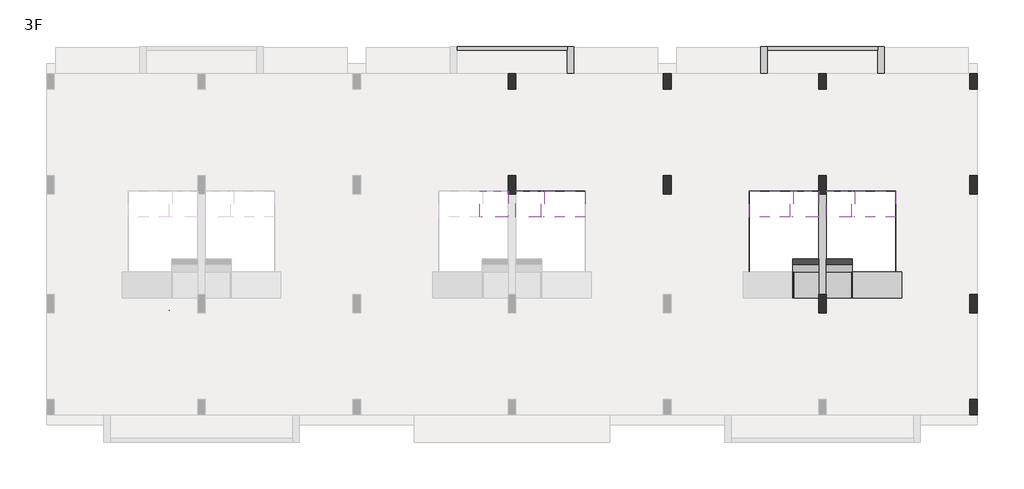
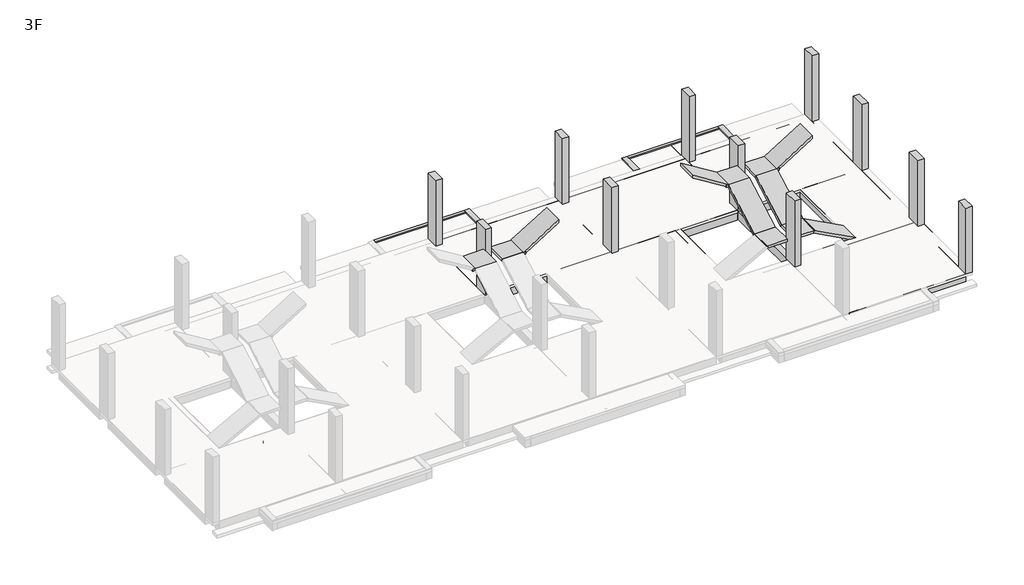
# One storey, part 3 of 3: 36 beams, 11 columns, 1 proxy.
"""IFC4 building model written with IfcOpenShell, lengths in millimetres."""

import ifcopenshell
import ifcopenshell.guid

model = None  # the IFC model being written
_history = None  # IfcOwnerHistory: only IFC2X3 demands one
_inside = {}  # id of a spatial element -> (the spatial element, [elements in it])
_under = {}  # id of a project, library or spatial element -> (it, [spatial elements below it])
_declared = {}  # id of a project -> (the project, [libraries it declares])
_typed = {}  # id of a type object -> (the type object, [elements of that type])
_made_of = {}  # id of a material, layer set ... -> (it, [elements and type objects made of it])


def new_model(schema):
    """Start an empty IFC model of exactly this schema.

    Asked for "IFC4X3", IfcOpenShell would pick the latest addendum, in which some entities
    have other attributes; the version numbers below select the first issue.
    IFC2X3 requires an IfcOwnerHistory on every rooted entity: one is made here for all.
    """
    global model, _history
    if schema == "IFC4X3":
        model = ifcopenshell.file(schema_version=(4, 3, 0, 0))
    else:
        model = ifcopenshell.file(schema=schema)
    _inside.clear()
    _under.clear()
    _declared.clear()
    _typed.clear()
    _made_of.clear()
    _history = None
    if model.schema == "IFC2X3":
        org = make("IfcOrganization", Name="unknown")
        user = make(
            "IfcPersonAndOrganization",
            ThePerson=make("IfcPerson", FamilyName="unknown"),
            TheOrganization=org,
        )
        app = make(
            "IfcApplication",
            ApplicationDeveloper=org,
            Version="unknown",
            ApplicationFullName="unknown",
            ApplicationIdentifier="unknown",
        )
        _history = make(
            "IfcOwnerHistory",
            OwningUser=user,
            OwningApplication=app,
            ChangeAction="ADDED",
            CreationDate=0,
        )
    return model


def make(cls, **values):
    """One entity of the class cls with the attributes given. An attribute that is None is left unset."""
    return model.create_entity(
        cls, **{name: value for name, value in values.items() if value is not None}
    )


def rooted(cls, **values):
    """An entity with a GlobalId (a new one), such as an element, a storey or a relation."""
    return make(cls, GlobalId=ifcopenshell.guid.new(), OwnerHistory=_history, **values)


def si_unit(unit_type, name, prefix=None):
    """IfcSIUnit, for example si_unit("LENGTHUNIT", "METRE", prefix="MILLI")."""
    return make("IfcSIUnit", UnitType=unit_type, Prefix=prefix, Name=name)


def assignment(units):
    """IfcUnitAssignment: the units of a project."""
    return None if units is None else make("IfcUnitAssignment", Units=units)


def point(xyz):
    """IfcCartesianPoint."""
    return None if xyz is None else make("IfcCartesianPoint", Coordinates=xyz)


def direction(xyz):
    """IfcDirection."""
    return None if xyz is None else make("IfcDirection", DirectionRatios=xyz)


def frame(location, z_axis=None, x_axis=None):
    """IfcAxis2Placement3D, a coordinate frame: its origin and axes. An axis left out is left unset."""
    return make(
        "IfcAxis2Placement3D",
        Location=point(location),
        Axis=direction(z_axis),
        RefDirection=direction(x_axis),
    )


def frame_2d(location, x_axis=None):
    """IfcAxis2Placement2D, a coordinate frame in the plane: its origin and x axis."""
    return make(
        "IfcAxis2Placement2D", Location=point(location), RefDirection=direction(x_axis)
    )


def origin():
    """The frame at (0, 0, 0) with its axes left unset."""
    return frame((0.0, 0.0, 0.0))


def origin_with_axes():
    """The frame at (0, 0, 0) with the z axis (0, 0, 1) and the x axis (1, 0, 0) written out."""
    return frame((0.0, 0.0, 0.0), z_axis=(0.0, 0.0, 1.0), x_axis=(1.0, 0.0, 0.0))


def place(relative_to, where):
    """IfcLocalPlacement: puts the frame where relative to a parent placement (None: the world)."""
    return make(
        "IfcLocalPlacement", PlacementRelTo=relative_to, RelativePlacement=where
    )


def context(
    kind, dimensions, precision=None, world=None, true_north=None, identifier=None
):
    """IfcGeometricRepresentationContext, for example the 3D "Model" context."""
    return make(
        "IfcGeometricRepresentationContext",
        ContextIdentifier=identifier,
        ContextType=kind,
        CoordinateSpaceDimension=dimensions,
        Precision=precision,
        WorldCoordinateSystem=world,
        TrueNorth=true_north,
    )


def project(units=None, contexts=None):
    """IfcProject with its units and contexts."""
    return rooted(
        "IfcProject",
        Name="project",
        RepresentationContexts=contexts,
        UnitsInContext=assignment(units),
    )


def spatial(cls, under=None, at=None, **own):
    """A site, building, storey or space (cls), placed at a placement, below another one or the project."""
    s = rooted(cls, ObjectPlacement=at, **own)
    if under is not None:
        _under.setdefault(under.id(), (under, []))[1].append(s)
    return s


def polyline(points):
    """IfcPolyline through the points."""
    return make("IfcPolyline", Points=[point(p) for p in points])


def circle_curve(where, radius):
    """IfcCircle in the frame where."""
    return make("IfcCircle", Position=where, Radius=radius)


def ellipse_curve(where, semi_axis1, semi_axis2):
    """IfcEllipse in the frame where."""
    return make(
        "IfcEllipse", Position=where, SemiAxis1=semi_axis1, SemiAxis2=semi_axis2
    )


def trimmed(basis, trim1, trim2, sense, master):
    """IfcTrimmedCurve: the piece of a basis curve between two trims."""
    return make(
        "IfcTrimmedCurve",
        BasisCurve=basis,
        Trim1=trim1,
        Trim2=trim2,
        SenseAgreement=sense,
        MasterRepresentation=master,
    )


def segment(curve, same_sense, transition):
    """IfcCompositeCurveSegment."""
    return make(
        "IfcCompositeCurveSegment",
        Transition=transition,
        SameSense=same_sense,
        ParentCurve=curve,
    )


def composite_curve(segments, self_intersect=None):
    """IfcCompositeCurve: segments joined end to end."""
    return make("IfcCompositeCurve", Segments=segments, SelfIntersect=self_intersect)


def outline(outer, holes=None, kind="AREA"):
    """IfcArbitraryClosedProfileDef: a profile drawn as a closed curve; with holes, ...WithVoids."""
    if holes is None:
        return make("IfcArbitraryClosedProfileDef", ProfileType=kind, OuterCurve=outer)
    return make(
        "IfcArbitraryProfileDefWithVoids",
        ProfileType=kind,
        OuterCurve=outer,
        InnerCurves=holes,
    )


def extrude(swept, where, along, depth):
    """IfcExtrudedAreaSolid: the profile swept, set in the frame where, extruded along a direction by depth."""
    return make(
        "IfcExtrudedAreaSolid",
        SweptArea=swept,
        Position=where,
        ExtrudedDirection=direction(along),
        Depth=depth,
    )


def faces_of(points, faces, orient=None, outer=None):
    """IfcFace entities. A face is a list of loops; a loop is a list of indices into points, from 0.

    orient and outer hold one flag for each loop. By default every Orientation is true, the
    first loop of a face is its IfcFaceOuterBound and the others are IfcFaceBound.
    """
    made = []
    for i, loops in enumerate(faces):
        bounds = []
        for j, loop in enumerate(loops):
            is_outer = j == 0 if outer is None else outer[i][j]
            bounds.append(
                make(
                    "IfcFaceOuterBound" if is_outer else "IfcFaceBound",
                    Bound=make("IfcPolyLoop", Polygon=[points[k] for k in loop]),
                    Orientation=True if orient is None else orient[i][j],
                )
            )
        made.append(make("IfcFace", Bounds=bounds))
    return made


def faceted_brep(points, faces, orient=None, outer=None, voids=None):
    """IfcFacetedBrep: a solid bounded by flat faces; with voids (closed shells), ...WithVoids."""
    shared = [point(p) for p in points]
    hull = make("IfcClosedShell", CfsFaces=faces_of(shared, faces, orient, outer))
    if voids is None:
        return make("IfcFacetedBrep", Outer=hull)
    return make(
        "IfcFacetedBrepWithVoids",
        Outer=hull,
        Voids=[
            make(cls, CfsFaces=faces_of(shared, fs, o, b)) for cls, fs, o, b in voids
        ],
    )


def shape(context_of_items, identifier, shape_type, items):
    """IfcShapeRepresentation: the items that make up one representation, for example the "Body"."""
    return make(
        "IfcShapeRepresentation",
        ContextOfItems=context_of_items,
        RepresentationIdentifier=identifier,
        RepresentationType=shape_type,
        Items=items,
    )


def source(mapping_origin, context_of_items, identifier, shape_type, items):
    """IfcRepresentationMap: a shape defined once, which mapped items show again and again."""
    return make(
        "IfcRepresentationMap",
        MappingOrigin=mapping_origin,
        MappedRepresentation=shape(context_of_items, identifier, shape_type, items),
    )


def transform(
    local_origin,
    x_axis=None,
    y_axis=None,
    z_axis=None,
    scale=None,
    scale2=None,
    scale3=None,
    uniform=True,
):
    """IfcCartesianTransformationOperator3D, or its non-uniform kind. x_axis, y_axis, z_axis: its Axis1, 2, 3."""
    if uniform:
        return make(
            "IfcCartesianTransformationOperator3D",
            Axis1=direction(x_axis),
            Axis2=direction(y_axis),
            LocalOrigin=point(local_origin),
            Scale=scale,
            Axis3=direction(z_axis),
        )
    return make(
        "IfcCartesianTransformationOperator3DnonUniform",
        Axis1=direction(x_axis),
        Axis2=direction(y_axis),
        LocalOrigin=point(local_origin),
        Scale=scale,
        Axis3=direction(z_axis),
        Scale2=scale2,
        Scale3=scale3,
    )


def mapped(mapping_source, mapping_target):
    """IfcMappedItem: shows the shape of a source again, moved by a transform."""
    return make(
        "IfcMappedItem", MappingSource=mapping_source, MappingTarget=mapping_target
    )


def made_of(thing, what):
    """Note that an element or type object is made of a material, layer set ...; save() writes the relation."""
    if what is not None:
        _made_of.setdefault(what.id(), (what, []))[1].append(thing)
    return thing


def element(
    cls,
    number,
    at=None,
    inside=None,
    cuts=None,
    type_object=None,
    material=None,
    context=None,
    identifier="Body",
    shape_type=None,
    held_by="IfcProductDefinitionShape",
    body=None,
    shapes=None,
    **own,
):
    """One element of the class cls, such as IfcWall. Its Tag is "e" and its number.

    at: its placement. inside: the storey or other place that contains it. cuts: it is an
    opening in that element (IfcRelVoidsElement). A single representation is given by context,
    identifier, shape_type and body (its items); several are given by shapes. held_by: the class
    of the entity that holds the representations. save() writes the other relations.
    """
    e = rooted(cls, Tag="e%d" % number, ObjectPlacement=at, **own)
    if body is not None:
        shapes = [shape(context, identifier, shape_type, body)]
    if shapes is not None:
        e.Representation = make(held_by, Representations=shapes)
    if inside is not None:
        _inside.setdefault(inside.id(), (inside, []))[1].append(e)
    if cuts is not None:
        rooted(
            "IfcRelVoidsElement", RelatingBuildingElement=cuts, RelatedOpeningElement=e
        )
    if type_object is not None:
        _typed.setdefault(type_object.id(), (type_object, []))[1].append(e)
    return made_of(e, material)


def aggregate(whole, parts):
    """IfcRelAggregates: a whole, such as a stair, and the parts it consists of."""
    return rooted("IfcRelAggregates", RelatingObject=whole, RelatedObjects=parts)


def save(model, path):
    """Write the relations noted so far, then the file.

    IfcRelAggregates (storeys below a building ...), IfcRelContainedInSpatialStructure (elements
    in a storey), IfcRelDefinesByType, IfcRelAssociatesMaterial and IfcRelDeclares: one each for
    every whole, place, type object, material and project.
    """
    for whole, parts in _under.values():
        aggregate(whole, parts)
    for where, things in _inside.values():
        rooted(
            "IfcRelContainedInSpatialStructure",
            RelatedElements=things,
            RelatingStructure=where,
        )
    for kind, things in _typed.values():
        rooted("IfcRelDefinesByType", RelatedObjects=things, RelatingType=kind)
    for what, things in _made_of.values():
        rooted("IfcRelAssociatesMaterial", RelatedObjects=things, RelatingMaterial=what)
    for by, libraries in _declared.values():
        rooted("IfcRelDeclares", RelatingContext=by, RelatedDefinitions=libraries)
    model.write(path)


def plane_surface(at):
    """IfcPlane: the flat surface through the origin of the frame at, square to its z axis."""
    return make("IfcPlane", Position=at)


def cylinder_surface(at, radius):
    """IfcCylindricalSurface: all points at the distance radius from the z axis of the frame at."""
    return make("IfcCylindricalSurface", Position=at, Radius=radius)


def revolved_surface(curve, axis_point, axis_direction):
    """IfcSurfaceOfRevolution: the curve turned about the line through axis_point along axis_direction."""
    return make(
        "IfcSurfaceOfRevolution",
        SweptCurve=make("IfcArbitraryOpenProfileDef", ProfileType="CURVE", Curve=curve),
        AxisPosition=make("IfcAxis1Placement", Location=point(axis_point), Axis=direction(axis_direction)),
    )


def advanced_brep(points, edges, surfaces, faces):
    """IfcAdvancedBrep: a solid bounded by faces that lie on surfaces and meet in shared edges.

    An edge is (start, end): straight between two places in points (the first is 0);
    or (start, end, curve); or (start, end, curve, False) where it runs against its curve.
    A face is (place in surfaces, loops), or (place, loops, False) where it looks against
    its surface's normal. A loop lists edges by number (the first is 1), with a minus sign
    where the edge is run from its end to its start. The first loop is the outer one.
    """
    corners = [point(p) for p in points]
    vertices = [make("IfcVertexPoint", VertexGeometry=c) for c in corners]
    made = []
    for start, end, *more in edges:
        made.append(
            make(
                "IfcEdgeCurve",
                EdgeStart=vertices[start],
                EdgeEnd=vertices[end],
                EdgeGeometry=more[0] if more else make("IfcPolyline", Points=[corners[start], corners[end]]),
                SameSense=more[1] if len(more) > 1 else True,
            )
        )
    hull = []
    for where, loops, *sense in faces:
        bounds = []
        for j, loop in enumerate(loops):
            ring = [make("IfcOrientedEdge", EdgeElement=made[abs(k) - 1], Orientation=k > 0) for k in loop]
            bounds.append(
                make(
                    "IfcFaceOuterBound" if j == 0 else "IfcFaceBound",
                    Bound=make("IfcEdgeLoop", EdgeList=ring),
                    Orientation=True,
                )
            )
        hull.append(make("IfcAdvancedFace", Bounds=bounds, FaceSurface=surfaces[where], SameSense=sense[0] if sense else True))
    return make("IfcAdvancedBrep", Outer=make("IfcClosedShell", CfsFaces=hull))


def m_support_metal_circular_m_support_metal_circular_a779fbb7(model_context):
    return source(origin(), model_context, "Body", "SolidModel", [
        advanced_brep(
        [(-6.0, 0.0, 0.0), (6.0, 0.0, 0.0), (-6.0, 0.0, -63.0), (6.0, 0.0, -63.0), (6.0, 12.0, -75.0), (-6.0, 12.0, -75.0), (-6.0, 63.0, -75.0), (6.0, 63.0, -75.0)],
        [
            (0, 1, circle_curve(origin_with_axes(), 6.0)),
            (1, 0, circle_curve(origin_with_axes(), 6.0)),
            (0, 2),
            (2, 3, circle_curve(frame((0.0, 0.0, -63.0), z_axis=(0.0, 0.0, 1.0), x_axis=(1.0, 0.0, 0.0)), 6.0)),
            (3, 1),
            (3, 2, circle_curve(frame((0.0, 0.0, -63.0), z_axis=(0.0, 0.0, 1.0), x_axis=(1.0, 0.0, 0.0)), 6.0)),
            (4, 3, circle_curve(frame((6.0, 12.0, -63.0), z_axis=(-1.0, 0.0, 0.0), x_axis=(0.0, -1.0, 0.0)), 12.0)),
            (2, 5, circle_curve(frame((-6.0, 12.0, -63.0), z_axis=(1.0, 0.0, 0.0), x_axis=(0.0, -1.0, 0.0)), 12.0)),
            (5, 4, circle_curve(frame((0.0, 12.0, -75.0), z_axis=(0.0, -1.0, 0.0), x_axis=(1.0, 0.0, 0.0)), 6.0)),
            (4, 5, circle_curve(frame((0.0, 12.0, -75.0), z_axis=(0.0, -1.0, 0.0), x_axis=(1.0, 0.0, 0.0)), 6.0)),
            (6, 7, circle_curve(frame((0.0, 63.0, -75.0), z_axis=(0.0, 1.0, 0.0), x_axis=(1.0, 0.0, 0.0)), 6.0)),
            (7, 6, circle_curve(frame((0.0, 63.0, -75.0), z_axis=(0.0, 1.0, 0.0), x_axis=(1.0, 0.0, 0.0)), 6.0)),
            (5, 6),
            (7, 4),
        ],
        [
            plane_surface(origin_with_axes()),
            cylinder_surface(origin_with_axes(), 6.0),
            revolved_surface(trimmed(ellipse_curve(frame((0.0, 0.0, -63.0), z_axis=(0.0, 0.0, 1.0), x_axis=(1.0, 0.0, 0.0)), 6.0, 6.0), [point((-6.0, 0.0, -63.0))], [point((6.0, 0.0, -63.0))], True, "CARTESIAN"), (0.0, 12.0, -63.0), (1.0, 0.0, 0.0)),
            revolved_surface(trimmed(ellipse_curve(frame((0.0, 0.0, -63.0), z_axis=(0.0, 0.0, 1.0), x_axis=(1.0, 0.0, 0.0)), 6.0, 6.0), [point((6.0, 0.0, -63.0))], [point((-6.0, 0.0, -63.0))], True, "CARTESIAN"), (0.0, 12.0, -63.0), (1.0, 0.0, 0.0)),
            plane_surface(frame((0.0, 63.0, -75.0), z_axis=(0.0, 1.0, 0.0), x_axis=(1.0, 0.0, 0.0))),
            cylinder_surface(frame((0.0, 12.0, -75.0), z_axis=(0.0, -1.0, 0.0), x_axis=(1.0, 0.0, 0.0)), 6.0),
        ],
        [
            (0, [[1, 2]]),
            (1, [[-1, 3, 4, 5]]),
            (1, [[-2, -5, 6, -3]]),
            (2, [[7, -4, 8, 9]]),
            (3, [[-8, -6, -7, 10]]),
            (4, [[11, 12]]),
            (5, [[-9, 13, -12, 14]]),
            (5, [[-10, -14, -11, -13]]),
        ],
    ),
        extrude(outline(composite_curve([segment(trimmed(circle_curve(frame_2d((-75.0, 0.0)), 25.0), [point((-75.0, -25.0))], [point((-75.0, 25.0))], False, "CARTESIAN"), True, "CONTINUOUS"), segment(trimmed(circle_curve(frame_2d((-75.0, 0.0)), 25.0), [point((-75.0, 25.0))], [point((-75.0, -25.0))], False, "CARTESIAN"), True, "CONTINUOUS")], self_intersect=False)), frame((0.0, 63.0, 0.0), z_axis=(0.0, 1.0, 0.0), x_axis=(0.0, 0.0, 1.0)), (0.0, 0.0, 1.0), 12.0),
    ])


model = new_model("IFC4")

# Units and contexts
model_context = context("Model", 3, world=origin())
ifc_project = project(units=[si_unit("LENGTHUNIT", "METRE", prefix="MILLI")], contexts=[model_context])

# Site, building, storey
site = spatial("IfcSite", under=ifc_project)
building = spatial("IfcBuilding", under=site)
storey = spatial("IfcBuildingStorey", under=building, Name="3F", Elevation=7330.0)

# Beams
placement = place(None, origin())
element("IfcBeam", 1, ObjectType="M_Concrete-Rectangular Beam : 1000x120", at=placement, inside=storey, context=model_context, shape_type="Brep", body=[
    faceted_brep([(16600.0000058, 7550.0000002, 9580.0), (16600.0000058, 8550.0000002, 9580.0), (16600.0000058, 8550.0000002, 9460.0), (16600.0000058, 7550.0000002, 9460.0), (17700.0000058, 8550.0000002, 9460.0), (17700.0000058, 8550.0000002, 9580.0), (17700.0000058, 7550.0000002, 9580.0), (17700.0000058, 7609.0063595, 9475.5095719), (17700.0000058, 7581.5414925, 9460.0), (16700.0000058, 7550.0000002, 9580.0), (16700.0000058, 7581.5414925, 9460.0), (16700.0000058, 7550.0000002, 9460.0), (16700.0000058, 7609.0063595, 9475.5095719)], [[[0, 1, 2, 3]], [[4, 5, 6, 7, 8]], [[1, 0, 9, 6, 5]], [[2, 1, 5, 4]], [[3, 2, 4, 8, 10, 11]], [[0, 3, 11, 9]], [[12, 7, 6, 9]], [[7, 12, 10, 8]], [[12, 9, 11, 10]]]),
])
element("IfcBeam", 2, ObjectType="M_Concrete-Rectangular Beam : 1000x120", at=placement, inside=storey, context=model_context, shape_type="Brep", body=[
    faceted_brep([(19100.0000058, 8550.0000002, 9580.0), (19100.0000058, 7550.0000002, 9580.0), (19100.0000058, 7550.0000002, 9460.0), (19100.0000058, 8550.0000002, 9460.0), (18000.0000058, 8550.0000002, 9580.0), (18000.0000058, 8550.0000002, 9460.0), (18000.0000058, 7581.5414925, 9460.0), (18000.0000058, 7609.0063595, 9475.5095719), (18000.0000058, 7550.0000002, 9580.0), (19000.0000058, 7550.0000002, 9580.0), (19000.0000058, 7550.0000002, 9460.0), (19000.0000058, 7581.5414925, 9460.0), (19000.0000058, 7609.0063595, 9475.5095719)], [[[0, 1, 2, 3]], [[4, 5, 6, 7, 8]], [[1, 0, 4, 8, 9]], [[0, 3, 5, 4]], [[3, 2, 10, 11, 6, 5]], [[2, 1, 9, 10]], [[12, 9, 8, 7]], [[12, 7, 6, 11]], [[9, 12, 11, 10]]]),
])
element("IfcBeam", 3, ObjectType="M_Concrete-Rectangular Beam : 1000x120", at=placement, inside=storey, context=model_context, shape_type="Brep", body=[
    faceted_brep([(18984.2496976, 7549.9999993, 9580.0), (20680.0000464, 7549.9999993, 10630.0), (20680.0000058, 8549.9999993, 10629.9999748), (18984.2496976, 8549.9999993, 9580.0), (20680.0000058, 8549.9999993, 10488.8582241), (19100.0000058, 8549.9999993, 9510.5302519), (19100.0000058, 8549.9999993, 9580.0), (19100.0000058, 7549.9999993, 9510.5302519), (20680.0000058, 7549.9999993, 10488.8582241), (19000.0000058, 7549.9999993, 9580.0), (19100.0000058, 7549.9999993, 9580.0)], [[[0, 1, 2, 3]], [[3, 2, 4, 5, 6]], [[7, 5, 4, 8]], [[1, 0, 9, 10, 7, 8]], [[10, 6, 5, 7]], [[6, 10, 9, 0, 3]], [[2, 1, 8, 4]]]),
])
element("IfcBeam", 4, ObjectType="M_Concrete-Rectangular Beam : 1000x120", at=placement, inside=storey, context=model_context, shape_type="Brep", body=[
    faceted_brep([(28700.0000039, 7550.0000002, 9580.0), (29700.0000039, 7550.0000002, 9580.0), (29700.0000039, 7609.0063595, 9475.5095719), (28700.0000039, 7609.0063595, 9475.5095719), (28700.0000039, 5424.9999998, 8380.0), (28700.0000039, 5484.0063591, 8275.5095719), (29700.0000039, 5484.0063591, 8275.5095719), (29700.0000039, 5424.9999998, 8380.0), (29700.0000039, 5524.9999998, 8298.6589219), (29700.0000039, 7581.5414925, 9460.0), (28700.0000039, 5524.9999998, 8298.6589219), (28700.0000039, 7581.5414925, 9460.0)], [[[0, 1, 2, 3]], [[4, 5, 6, 7]], [[1, 0, 4, 7]], [[2, 1, 7, 6, 8, 9]], [[3, 2, 9, 8, 6, 5, 10, 11]], [[0, 3, 11, 10, 5, 4]]]),
])
element("IfcBeam", 5, ObjectType="M_Concrete-Rectangular Beam : 1000x120", at=placement, inside=storey, context=model_context, shape_type="Brep", body=[
    faceted_brep([(28600.0000039, 7550.0000002, 9580.0), (28600.0000039, 8550.0000002, 9580.0), (28600.0000039, 8550.0000002, 9460.0), (28600.0000039, 7550.0000002, 9460.0), (29700.0000039, 8550.0000002, 9460.0), (29700.0000039, 8550.0000002, 9580.0), (29700.0000039, 7550.0000002, 9580.0), (29700.0000039, 7609.0063595, 9475.5095719), (29700.0000039, 7581.5414925, 9460.0), (28700.0000039, 7550.0000002, 9580.0), (28700.0000039, 7581.5414925, 9460.0), (28700.0000039, 7550.0000002, 9460.0), (28700.0000039, 7609.0063595, 9475.5095719)], [[[0, 1, 2, 3]], [[4, 5, 6, 7, 8]], [[1, 0, 9, 6, 5]], [[2, 1, 5, 4]], [[3, 2, 4, 8, 10, 11]], [[0, 3, 11, 9]], [[12, 7, 6, 9]], [[7, 12, 10, 8]], [[12, 9, 11, 10]]]),
])
element("IfcBeam", 6, ObjectType="M_Concrete-Rectangular Beam : 1000x120", at=placement, inside=storey, context=model_context, shape_type="Brep", body=[
    faceted_brep([(27019.9999632, 7549.9999993, 10630.0), (28715.750312, 7549.9999993, 9580.0), (28715.750312, 8549.9999993, 9580.0), (27019.9999632, 8549.9999993, 10630.0), (28600.0000039, 8549.9999993, 9580.0), (28600.0000039, 8549.9999993, 9510.5302519), (27020.000004, 8549.9999993, 10488.8582239), (28600.0000039, 7549.9999993, 9510.5302519), (27020.000004, 7549.9999993, 10488.8582239), (28600.0000039, 7549.9999993, 9580.0), (28700.0000039, 7549.9999993, 9580.0)], [[[0, 1, 2, 3]], [[3, 2, 4, 5, 6]], [[5, 7, 8, 6]], [[1, 0, 8, 7, 9, 10]], [[4, 9, 7, 5]], [[9, 4, 2, 1, 10]], [[0, 3, 6, 8]]]),
])
element("IfcBeam", 7, ObjectType="M_Concrete-Rectangular Beam : 1000x120", at=placement, inside=storey, context=model_context, shape_type="Brep", body=[
    faceted_brep([(29700.0000039, 5524.9999998, 8260.0), (28700.0000039, 5524.9999998, 8260.0), (28700.0000039, 5524.9999998, 8298.6589219), (29700.0000039, 5524.9999998, 8298.6589219), (29700.0000039, 4424.9999998, 8260.0), (29700.0000039, 4424.9999998, 8380.0), (28730.4772098, 4424.9999998, 8380.0), (28787.1330609, 4424.9999998, 8274.2166623), (28760.5888301, 4424.9999998, 8260.0), (29700.0000039, 5424.9999998, 8380.0), (28700.0000039, 5424.9999998, 8380.0), (28700.0000039, 4424.9999998, 8380.0), (29700.0000039, 5484.0063591, 8275.5095719), (28760.5888301, 5424.9999998, 8260.0), (28700.0000039, 5424.9999998, 8260.0), (28700.0000039, 4424.9999998, 8363.6768996), (28700.0000039, 5484.0063591, 8275.5095719), (28700.0000039, 5424.9999998, 8363.6768996), (28730.4772098, 5424.9999998, 8380.0), (28787.1330609, 5424.9999998, 8274.2166623)], [[[0, 1, 2, 3]], [[4, 5, 6, 7, 8]], [[6, 5, 9, 10, 11]], [[5, 4, 0, 3, 12, 9]], [[1, 0, 4, 8, 13, 14]], [[15, 11, 10, 16, 2, 1, 14, 17]], [[6, 18, 19, 7]], [[18, 6, 15, 17]], [[7, 19, 13, 8]], [[19, 18, 17, 14, 13]], [[11, 15, 6]], [[12, 16, 10, 9]], [[16, 12, 3, 2]]]),
])
element("IfcBeam", 8, ObjectType="M_Concrete-Rectangular Beam : 1000x120", at=placement, inside=storey, context=model_context, shape_type="Brep", body=[
    faceted_brep([(30969.5227979, 4424.9999998, 8380.0), (30969.5227979, 5424.9999998, 8380.0), (30912.8669468, 5424.9999998, 8274.2166623), (30912.8669468, 4424.9999998, 8274.2166623), (31000.0000039, 4424.9999998, 8363.6768996), (32930.0000046, 4424.9999998, 7330.0), (32930.0000046, 5424.9999998, 7330.0), (31000.0000039, 5424.9999998, 8363.6768996), (30939.4111776, 4424.9999998, 8260.0), (32675.8338464, 4424.9999998, 7330.0), (30939.4111776, 5424.9999998, 8260.0), (32680.0000108, 5424.9999998, 7327.7686695), (32680.0000108, 4449.9999998, 7327.7686695), (32675.8338464, 4449.9999998, 7330.0), (32680.0000108, 5424.9999998, 7330.0), (32680.0000108, 4449.9999998, 7330.0)], [[[0, 1, 2, 3]], [[1, 0, 4, 5, 6, 7]], [[0, 3, 8, 9, 5, 4]], [[3, 2, 10, 11, 12, 13, 9, 8]], [[2, 1, 7, 6, 14, 11, 10]], [[9, 13, 15, 14, 6, 5]], [[11, 14, 15, 12]], [[15, 13, 12]]]),
])
element("IfcBeam", 9, ObjectType="M_Concrete-Rectangular Beam : 1000x120", at=placement, inside=storey, context=model_context, shape_type="Brep", body=[
    faceted_brep([(31000.0000039, 7550.0000002, 9580.0), (31000.0000039, 7609.0063595, 9475.5095719), (30000.0000039, 7609.0063595, 9475.5095719), (30000.0000039, 7550.0000002, 9580.0), (31000.0000039, 5424.9999998, 8380.0), (30000.0000039, 5424.9999998, 8380.0), (30000.0000039, 5484.0063591, 8275.5095719), (31000.0000039, 5484.0063591, 8275.5095719), (30000.0000039, 7581.5414925, 9460.0), (30000.0000039, 5524.9999998, 8298.6589219), (31000.0000039, 7581.5414925, 9460.0), (31000.0000039, 5524.9999998, 8298.6589219)], [[[0, 1, 2, 3]], [[4, 5, 6, 7]], [[3, 5, 4, 0]], [[2, 8, 9, 6, 5, 3]], [[1, 10, 11, 7, 6, 9, 8, 2]], [[0, 4, 7, 11, 10, 1]]]),
])
element("IfcBeam", 10, ObjectType="M_Concrete-Rectangular Beam : 1000x120", at=placement, inside=storey, context=model_context, shape_type="Brep", body=[
    faceted_brep([(31100.0000039, 8550.0000002, 9580.0), (31100.0000039, 7550.0000002, 9580.0), (31100.0000039, 7550.0000002, 9460.0), (31100.0000039, 8550.0000002, 9460.0), (30000.0000039, 8550.0000002, 9580.0), (30000.0000039, 8550.0000002, 9460.0), (30000.0000039, 7581.5414925, 9460.0), (30000.0000039, 7609.0063595, 9475.5095719), (30000.0000039, 7550.0000002, 9580.0), (31000.0000039, 7550.0000002, 9580.0), (31000.0000039, 7550.0000002, 9460.0), (31000.0000039, 7581.5414925, 9460.0), (31000.0000039, 7609.0063595, 9475.5095719)], [[[0, 1, 2, 3]], [[4, 5, 6, 7, 8]], [[1, 0, 4, 8, 9]], [[0, 3, 5, 4]], [[3, 2, 10, 11, 6, 5]], [[2, 1, 9, 10]], [[12, 9, 8, 7]], [[12, 7, 6, 11]], [[9, 12, 11, 10]]]),
])
element("IfcBeam", 11, ObjectType="M_Concrete-Rectangular Beam : 1000x120", at=placement, inside=storey, context=model_context, shape_type="Brep", body=[
    faceted_brep([(30984.2496957, 7549.9999993, 9580.0), (32680.0000445, 7549.9999993, 10630.0), (32680.0000108, 8549.9999993, 10629.9999791), (30984.2496957, 8549.9999993, 9580.0), (32680.0000108, 8549.9999993, 10488.8582284), (31100.0000039, 8549.9999993, 9510.5302519), (31100.0000039, 8549.9999993, 9580.0), (31100.0000039, 7549.9999993, 9510.5302519), (32680.0000108, 7549.9999993, 10488.8582284), (31000.0000039, 7549.9999993, 9580.0), (31100.0000039, 7549.9999993, 9580.0)], [[[0, 1, 2, 3]], [[3, 2, 4, 5, 6]], [[7, 5, 4, 8]], [[1, 0, 9, 10, 7, 8]], [[10, 6, 5, 7]], [[6, 10, 9, 0, 3]], [[2, 1, 8, 4]]]),
])
element("IfcBeam", 12, ObjectType="M_Concrete-Rectangular Beam : 1000x120", at=placement, inside=storey, context=model_context, shape_type="Brep", body=[
    faceted_brep([(31000.0000039, 5524.9999998, 8260.0), (30000.0000039, 5524.9999998, 8260.0), (30000.0000039, 5524.9999998, 8298.6589219), (31000.0000039, 5524.9999998, 8298.6589219), (30000.0000039, 4424.9999998, 8380.0), (30000.0000039, 4424.9999998, 8260.0), (30939.4111776, 4424.9999998, 8260.0), (30912.8669468, 4424.9999998, 8274.2166623), (30969.5227979, 4424.9999998, 8380.0), (31000.0000039, 4424.9999998, 8380.0), (31000.0000039, 5424.9999998, 8380.0), (30000.0000039, 5424.9999998, 8380.0), (30000.0000039, 5484.0063591, 8275.5095719), (31000.0000039, 5424.9999998, 8260.0), (30939.4111776, 5424.9999998, 8260.0), (31000.0000039, 4424.9999998, 8363.6768996), (31000.0000039, 5424.9999998, 8363.6768996), (31000.0000039, 5484.0063591, 8275.5095719), (30969.5227979, 5424.9999998, 8380.0), (30912.8669468, 5424.9999998, 8274.2166623)], [[[0, 1, 2, 3]], [[4, 5, 6, 7, 8]], [[8, 9, 10, 11, 4]], [[5, 4, 11, 12, 2, 1]], [[1, 0, 13, 14, 6, 5]], [[9, 15, 16, 13, 0, 3, 17, 10]], [[18, 8, 7, 19]], [[8, 18, 16, 15]], [[19, 7, 6, 14]], [[18, 19, 14, 13, 16]], [[15, 9, 8]], [[17, 12, 11, 10]], [[12, 17, 3, 2]]]),
])
element("IfcBeam", 13, ObjectType="M_Concrete-Rectangular Beam : 150x500", at=placement, inside=storey, context=model_context, shape_type="SweptSolid", body=[
    extrude(outline(polyline([(19989.9825383, 14150.0000066), (19989.9825383, 14000.0000066), (15710.0998466, 14000.0000066), (15710.0998466, 14150.0000066), (19989.9825383, 14150.0000066)])), frame((0.0, 0.0, 6830.0), z_axis=(0.0, 0.0, 1.0), x_axis=(1.0, 0.0, 0.0)), (0.0, 0.0, 1.0), 500.0),
])
element("IfcBeam", 14, ObjectType="M_Concrete-Rectangular Beam : 150x500", at=placement, inside=storey, context=model_context, shape_type="SweptSolid", body=[
    extrude(outline(polyline([(31989.900241, 14150.0000066), (31989.900241, 14000.0000066), (27710.0128711, 14000.0000066), (27710.0128711, 14150.0000066), (31989.900241, 14150.0000066)])), frame((0.0, 0.0, 6830.0), z_axis=(0.0, 0.0, 1.0), x_axis=(1.0, 0.0, 0.0)), (0.0, 0.0, 1.0), 500.0),
])
element("IfcBeam", 15, ObjectType="M_Concrete-Rectangular Beam : 250x400", at=placement, inside=storey, context=model_context, shape_type="Brep", body=[
    faceted_brep([(32930.0000108, 8549.9999993, 7330.0), (32680.0000108, 8549.9999993, 7330.0), (32680.0000108, 5424.9999998, 7330.0), (32680.0000108, 4449.9999998, 7330.0), (32930.0000108, 4449.9999998, 7330.0), (32930.0000108, 8549.9999993, 6930.0), (32930.0000108, 4449.9999998, 6930.0), (32680.0000108, 8549.9999993, 6930.0), (32680.0000108, 4449.9999998, 6930.0), (32680.0000108, 8549.9999993, 7188.8582284), (32680.0000108, 4449.9999998, 7327.7686695)], [[[0, 1, 2, 3, 4]], [[5, 0, 4, 6]], [[7, 5, 6, 8]], [[1, 9, 7, 8, 10, 3, 2]], [[1, 0, 5, 7, 9]], [[4, 3, 10, 8, 6]]]),
])
element("IfcBeam", 16, ObjectType="M_Concrete-Rectangular Beam : 250x400", at=placement, inside=storey, context=model_context, shape_type="Brep", body=[
    faceted_brep([(27020.000004, 8549.9999993, 7330.0), (26770.000004, 8549.9999993, 7330.0), (26770.000004, 4449.9999998, 7330.0), (27020.000004, 4449.9999998, 7330.0), (27020.000004, 5424.9999998, 7330.0), (27020.000004, 8549.9999993, 6930.0), (27020.000004, 8549.9999993, 7188.8582239), (27020.000004, 4449.9999998, 7327.7686733), (27020.000004, 4449.9999998, 6930.0), (26770.000004, 8549.9999993, 6930.0), (26770.000004, 4449.9999998, 6930.0)], [[[0, 1, 2, 3, 4]], [[5, 6, 0, 4, 3, 7, 8]], [[9, 5, 8, 10]], [[1, 9, 10, 2]], [[1, 0, 6, 5, 9]], [[3, 2, 10, 8, 7]]]),
])
element("IfcBeam", 17, ObjectType="M_Concrete-Rectangular Beam : 250x500", at=placement, inside=storey, context=model_context, shape_type="Brep", body=[
    faceted_brep([(20239.9825383, 14150.0000066, 7330.0), (19989.9825383, 14150.0000066, 7330.0), (19989.9825383, 14000.0000066, 7330.0), (19989.9825383, 13100.0000001, 7330.0), (20239.9825383, 13100.0000001, 7330.0), (19989.9825383, 14150.0000066, 6830.0), (19989.9825383, 14000.0000066, 6830.0), (19989.9825383, 13100.0000001, 6830.0), (20239.9825383, 14150.0000066, 6830.0), (20239.9825383, 13100.0000001, 6830.0)], [[[0, 1, 2, 3, 4]], [[1, 5, 6, 7, 3, 2]], [[5, 8, 9, 7, 6]], [[8, 0, 4, 9]], [[1, 0, 8, 5]], [[4, 3, 7, 9]]]),
])
element("IfcBeam", 18, ObjectType="M_Concrete-Rectangular Beam : 250x500", at=placement, inside=storey, context=model_context, shape_type="Brep", body=[
    faceted_brep([(32239.900241, 14150.0000066, 7330.0), (31989.900241, 14150.0000066, 7330.0), (31989.900241, 14000.0000066, 7330.0), (31989.900241, 13100.0000001, 7330.0), (32239.900241, 13100.0000001, 7330.0), (31989.900241, 14150.0000066, 6830.0), (31989.900241, 14000.0000066, 6830.0), (31989.900241, 13100.0000001, 6830.0), (32239.900241, 14150.0000066, 6830.0), (32239.900241, 13100.0000001, 6830.0)], [[[0, 1, 2, 3, 4]], [[1, 5, 6, 7, 3, 2]], [[5, 8, 9, 7, 6]], [[8, 0, 4, 9]], [[4, 3, 7, 9]], [[1, 0, 8, 5]]]),
])
element("IfcBeam", 19, ObjectType="M_Concrete-Rectangular Beam : 250x500", at=placement, inside=storey, context=model_context, shape_type="Brep", body=[
    faceted_brep([(27710.0128711, 14150.0000066, 7330.0), (27460.0128711, 14150.0000066, 7330.0), (27460.0128711, 13100.0000001, 7330.0), (27710.0128711, 13100.0000001, 7330.0), (27710.0128711, 14000.0000066, 7330.0), (27710.0128711, 14150.0000066, 6830.0), (27710.0128711, 13100.0000001, 6830.0), (27710.0128711, 14000.0000066, 6830.0), (27460.0128711, 14150.0000066, 6830.0), (27460.0128711, 13100.0000001, 6830.0)], [[[0, 1, 2, 3, 4]], [[5, 0, 4, 3, 6, 7]], [[8, 5, 7, 6, 9]], [[1, 8, 9, 2]], [[3, 2, 9, 6]], [[1, 0, 5, 8]]]),
])
element("IfcBeam", 20, ObjectType="M_Concrete-Rectangular Beam : 300x400", at=placement, inside=storey, context=model_context, shape_type="SweptSolid", body=[
    extrude(outline(polyline([(18000.0000046, 9150.0), (17700.0000046, 9150.0), (17700.0000046, 12500.0000003), (18000.0000046, 12500.0000003), (18000.0000046, 9150.0)])), frame((0.0, 0.0, 6930.0), z_axis=(0.0, 0.0, 1.0), x_axis=(1.0, 0.0, 0.0)), (0.0, 0.0, 1.0), 400.0),
])
element("IfcBeam", 21, ObjectType="M_Concrete-Rectangular Beam : 300x400", at=placement, inside=storey, context=model_context, shape_type="SweptSolid", body=[
    extrude(outline(polyline([(30000.0000031, 9149.9985388), (29700.0000031, 9149.9985388), (29700.0000031, 12500.0000003), (30000.0000031, 12500.0000003), (30000.0000031, 9149.9985388)])), frame((0.0, 0.0, 6930.0), z_axis=(0.0, 0.0, 1.0), x_axis=(1.0, 0.0, 0.0)), (0.0, 0.0, 1.0), 400.0),
])
element("IfcBeam", 22, ObjectType="M_Concrete-Rectangular Beam : 300x400", at=placement, inside=storey, context=model_context, shape_type="SweptSolid", body=[
    extrude(outline(polyline([(30000.0000031, 4550.0000002), (29700.0000031, 4550.0000002), (29700.0000031, 8449.9985388), (30000.0000031, 8449.9985388), (30000.0000031, 4550.0000002)])), frame((0.0, 0.0, 6930.0), z_axis=(0.0, 0.0, 1.0), x_axis=(1.0, 0.0, 0.0)), (0.0, 0.0, 1.0), 400.0),
])
element("IfcBeam", 23, ObjectType="M_Concrete-Rectangular Beam : 300x400", at=placement, inside=storey, context=model_context, shape_type="SweptSolid", body=[
    extrude(outline(polyline([(35835.035019, 9149.9985388), (35535.035019, 9149.9985388), (35535.035019, 12500.0000003), (35835.035019, 12500.0000003), (35835.035019, 9149.9985388)])), frame((0.0, 0.0, 6930.0), z_axis=(0.0, 0.0, 1.0), x_axis=(1.0, 0.0, 0.0)), (0.0, 0.0, 1.0), 400.0),
])
element("IfcBeam", 24, ObjectType="M_Concrete-Rectangular Beam : 300x400", at=placement, inside=storey, context=model_context, shape_type="SweptSolid", body=[
    extrude(outline(polyline([(35835.035019, 4550.0000002), (35535.035019, 4550.0000002), (35535.035019, 8449.9985388), (35835.035019, 8449.9985388), (35835.035019, 4550.0000002)])), frame((0.0, 0.0, 6930.0), z_axis=(0.0, 0.0, 1.0), x_axis=(1.0, 0.0, 0.0)), (0.0, 0.0, 1.0), 400.0),
])
element("IfcBeam", 25, ObjectType="M_Concrete-Rectangular Beam : 300x400", at=placement, inside=storey, context=model_context, shape_type="SweptSolid", body=[
    extrude(outline(polyline([(35835.035019, 499.9999998), (35535.035019, 499.9999998), (35535.035019, 3850.0000002), (35835.035019, 3850.0000002), (35835.035019, 499.9999998)])), frame((0.0, 0.0, 6930.0), z_axis=(0.0, 0.0, 1.0), x_axis=(1.0, 0.0, 0.0)), (0.0, 0.0, 1.0), 400.0),
])
element("IfcBeam", 26, ObjectType="M_Concrete-Rectangular Beam : 300x400", at=placement, inside=storey, context=model_context, shape_type="SweptSolid", body=[
    extrude(outline(polyline([(24000.000004, 9149.9985388), (23700.000004, 9149.9985388), (23700.000004, 12500.0000003), (24000.000004, 12500.0000003), (24000.000004, 9149.9985388)])), frame((0.0, 0.0, 6930.0), z_axis=(0.0, 0.0, 1.0), x_axis=(1.0, 0.0, 0.0)), (0.0, 0.0, 1.0), 400.0),
])
element("IfcBeam", 27, ObjectType="M_Concrete-Rectangular Beam : 300x400", at=placement, inside=storey, context=model_context, shape_type="SweptSolid", body=[
    extrude(outline(polyline([(18000.0064311, 13100.0000003), (17700.0064311, 13100.0000001), (17700.0064311, 14000.0000066), (18000.0064311, 14000.0000066), (18000.0064311, 13100.0000003)])), frame((0.0, 0.0, 6880.0), z_axis=(0.0, 0.0, 1.0), x_axis=(1.0, 0.0, 0.0)), (0.0, 0.0, 1.0), 400.0),
])
element("IfcBeam", 28, ObjectType="M_Concrete-Rectangular Beam : 300x400", at=placement, inside=storey, context=model_context, shape_type="SweptSolid", body=[
    extrude(outline(polyline([(30000.0064292, 13100.0000003), (29700.0064292, 13100.0000001), (29700.0064292, 14000.0000066), (30000.0064292, 14000.0000066), (30000.0064292, 13100.0000003)])), frame((0.0, 0.0, 6880.0), z_axis=(0.0, 0.0, 1.0), x_axis=(1.0, 0.0, 0.0)), (0.0, 0.0, 1.0), 400.0),
])
element("IfcBeam", 29, ObjectType="M_Concrete-Rectangular Beam : 300x500", at=placement, inside=storey, context=model_context, shape_type="Brep", body=[
    faceted_brep([(18000.0000058, 13100.0000001, 7330.0), (18000.0000058, 12800.0000001, 7330.0), (23700.0000047, 12800.0000001, 7330.0), (23700.0000047, 13100.0000001, 7330.0), (20239.9825383, 13100.0000001, 7330.0), (19989.9825383, 13100.0000001, 7330.0), (18000.0000058, 12800.0000001, 6830.0), (23700.0000047, 12800.0000001, 6830.0), (18000.0000058, 13100.0000001, 6830.0), (19989.9825383, 13100.0000001, 6830.0), (20239.9825383, 13100.0000001, 6830.0), (23700.0000047, 13100.0000001, 6830.0)], [[[0, 1, 2, 3, 4, 5]], [[1, 6, 7, 2]], [[6, 8, 9, 10, 11, 7]], [[8, 0, 5, 4, 3, 11, 10, 9]], [[1, 0, 8, 6]], [[3, 2, 7, 11]]]),
])
element("IfcBeam", 30, ObjectType="M_Concrete-Rectangular Beam : 300x500", at=placement, inside=storey, context=model_context, shape_type="Brep", body=[
    faceted_brep([(18000.0000058, 8849.9999993, 7330.0), (18000.0000058, 8549.9999993, 7330.0), (20680.0000058, 8549.9999993, 7330.0), (20930.0000058, 8549.9999993, 7330.0), (23700.0000047, 8549.9999993, 7330.0), (23700.0000047, 8849.9999993, 7330.0), (18000.0000058, 8549.9999993, 6830.0), (23700.0000047, 8549.9999993, 6830.0), (18000.0000058, 8849.9999993, 6830.0), (23700.0000047, 8849.9999993, 6830.0)], [[[0, 1, 2, 3, 4, 5]], [[1, 6, 7, 4, 3, 2]], [[6, 8, 9, 7]], [[8, 0, 5, 9]], [[1, 0, 8, 6]], [[5, 4, 7, 9]]]),
])
element("IfcBeam", 31, ObjectType="M_Concrete-Rectangular Beam : 300x500", at=placement, inside=storey, context=model_context, shape_type="Brep", body=[
    faceted_brep([(24000.0000047, 13100.0000001, 7330.0), (24000.000004, 12800.0000001, 7330.0), (29700.0000039, 12800.0000001, 7330.0), (29700.0000039, 13100.0000001, 7330.0), (27710.0128711, 13100.0000001, 7330.0), (27460.0128711, 13100.0000001, 7330.0), (24000.0000047, 12800.0000001, 6830.0), (29700.0000039, 12800.0000001, 6830.0), (24000.0000047, 13100.0000001, 6830.0), (27460.0128711, 13100.0000001, 6830.0), (27710.0128711, 13100.0000001, 6830.0), (29700.0000039, 13100.0000001, 6830.0)], [[[0, 1, 2, 3, 4, 5]], [[1, 6, 7, 2]], [[6, 8, 9, 10, 11, 7]], [[8, 0, 5, 4, 3, 11, 10, 9]], [[8, 6, 1, 0]], [[3, 2, 7, 11]]]),
])
element("IfcBeam", 32, ObjectType="M_Concrete-Rectangular Beam : 300x500", at=placement, inside=storey, context=model_context, shape_type="Brep", body=[
    faceted_brep([(24000.000004, 8849.9999993, 7330.0), (24000.0000047, 8549.9999993, 7330.0), (26770.000004, 8549.9999993, 7330.0), (27020.000004, 8549.9999993, 7330.0), (29700.0000039, 8549.9999993, 7330.0), (29700.0000039, 8849.9999993, 7330.0), (24000.0000047, 8549.9999993, 6830.0), (29700.0000039, 8549.9999993, 6830.0), (24000.0000047, 8849.9999993, 6830.0), (29700.0000039, 8849.9999993, 6830.0)], [[[0, 1, 2, 3, 4, 5]], [[1, 6, 7, 4, 3, 2]], [[6, 8, 9, 7]], [[8, 0, 5, 9]], [[6, 1, 0, 8]], [[5, 4, 7, 9]]]),
])
element("IfcBeam", 33, ObjectType="M_Concrete-Rectangular Beam : 300x500", at=placement, inside=storey, context=model_context, shape_type="Brep", body=[
    faceted_brep([(30000.0000039, 13100.0000001, 7330.0), (30000.0000039, 12800.0000001, 7330.0), (35535.035019, 12800.0000001, 7330.0), (35535.035019, 13100.0000001, 7330.0), (32239.900241, 13100.0000001, 7330.0), (31989.900241, 13100.0000001, 7330.0), (30000.0000039, 12800.0000001, 6830.0), (35535.035019, 12800.0000001, 6830.0), (30000.0000039, 13100.0000001, 6830.0), (31989.900241, 13100.0000001, 6830.0), (32239.900241, 13100.0000001, 6830.0), (35535.035019, 13100.0000001, 6830.0)], [[[0, 1, 2, 3, 4, 5]], [[1, 6, 7, 2]], [[6, 8, 9, 10, 11, 7]], [[8, 0, 5, 4, 3, 11, 10, 9]], [[1, 0, 8, 6]], [[3, 2, 7, 11]]]),
])
element("IfcBeam", 34, ObjectType="M_Concrete-Rectangular Beam : 300x500", at=placement, inside=storey, context=model_context, shape_type="Brep", body=[
    faceted_brep([(30000.0000039, 8849.9999993, 7330.0), (30000.0000039, 8549.9999993, 7330.0), (32680.0000108, 8549.9999993, 7330.0), (32930.0000108, 8549.9999993, 7330.0), (35535.035019, 8549.9999993, 7330.0), (35535.035019, 8849.9999993, 7330.0), (30000.0000039, 8549.9999993, 6830.0), (35535.035019, 8549.9999993, 6830.0), (30000.0000039, 8849.9999993, 6830.0), (35535.035019, 8849.9999993, 6830.0)], [[[0, 1, 2, 3, 4, 5]], [[1, 6, 7, 4, 3, 2]], [[6, 8, 9, 7]], [[8, 0, 5, 9]], [[1, 0, 8, 6]], [[5, 4, 7, 9]]]),
])
element("IfcBeam", 35, ObjectType="M_Concrete-Rectangular Beam : 300x500", at=placement, inside=storey, context=model_context, shape_type="Brep", body=[
    faceted_brep([(30000.0000031, 4449.9999998, 7330.0), (30000.0000031, 4149.9999998, 7330.0), (35535.035019, 4149.9999998, 7330.0), (35535.035019, 4449.9999998, 7330.0), (32930.0000108, 4449.9999998, 7330.0), (32680.0000108, 4449.9999998, 7330.0), (32675.8338464, 4449.9999998, 7330.0), (30000.0000039, 4149.9999998, 6830.0), (35535.035019, 4149.9999998, 6830.0), (30000.0000039, 4449.9999998, 6830.0), (35535.035019, 4449.9999998, 6830.0)], [[[0, 1, 2, 3, 4, 5, 6]], [[1, 7, 8, 2]], [[7, 9, 10, 8]], [[9, 0, 6, 5, 4, 3, 10]], [[1, 0, 9, 7]], [[3, 2, 8, 10]]]),
])
element("IfcBeam", 36, ObjectType="M_Concrete-Rectangular Beam : 300x500", at=placement, inside=storey, context=model_context, shape_type="Brep", body=[
    faceted_brep([(30000.0000039, 202.2719854, 7330.0), (30000.0000039, -97.7280146, 7330.0), (33380.0128581, -97.7280146, 7330.0), (33630.0128581, -97.7280146, 7330.0), (35535.035019, -97.7280146, 7330.0), (35535.035019, 202.2719854, 7330.0), (30000.0000039, -97.7280146, 6830.0), (33380.0128581, -97.7280146, 6830.0), (33630.0128581, -97.7280146, 6830.0), (35535.035019, -97.7280146, 6830.0), (30000.0000039, 202.2719854, 6830.0), (35535.035019, 202.2719854, 6830.0)], [[[0, 1, 2, 3, 4, 5]], [[1, 6, 7, 8, 9, 4, 3, 2]], [[6, 10, 11, 9, 8, 7]], [[10, 0, 5, 11]], [[1, 0, 10, 6]], [[5, 4, 9, 11]]]),
])

# Proxy
m_support_metal_circular_m_support_metal_circular_shape = m_support_metal_circular_m_support_metal_circular_a779fbb7(model_context)
element("IfcBuildingElementProxy", 37, Name="M_Support - Metal - Circular : M_Support - Metal - Circular", ObjectType="M_Support - Metal - Circular : M_Support - Metal - Circular", at=placement, inside=storey, context=model_context, shape_type="MappedRepresentation", body=[
    mapped(m_support_metal_circular_m_support_metal_circular_shape, transform((4604.999959, 3949.9999996, 7330.0), x_axis=(1.0, 0.0, 0.0), y_axis=(0.0, 1.0, 0.0), z_axis=(0.0, 0.0, 1.0))),
])

# Columns
element("IfcColumn", 38, ObjectType="M_Concrete-Rectangular-Column : 300x600", at=placement, inside=storey, context=model_context, shape_type="SweptSolid", body=[
    extrude(outline(polyline([(18000.0000058, 13100.0000005), (18000.0000058, 12500.0000005), (17700.0000058, 12500.0000005), (17700.0000058, 13100.0000005), (18000.0000058, 13100.0000005)])), frame((0.0, 0.0, 7330.0), z_axis=(0.0, 0.0, 1.0), x_axis=(1.0, 0.0, 0.0)), (0.0, 0.0, 1.0), 3300.0),
])
element("IfcColumn", 39, ObjectType="M_Concrete-Rectangular-Column : 300x600", at=placement, inside=storey, context=model_context, shape_type="SweptSolid", body=[
    extrude(outline(polyline([(24000.0000047, 13100.0000005), (24000.0000047, 12500.0000005), (23700.0000047, 12500.0000005), (23700.0000047, 13100.0000005), (24000.0000047, 13100.0000005)])), frame((0.0, 0.0, 7330.0), z_axis=(0.0, 0.0, 1.0), x_axis=(1.0, 0.0, 0.0)), (0.0, 0.0, 1.0), 3300.0),
])
element("IfcColumn", 40, ObjectType="M_Concrete-Rectangular-Column : 300x600", at=placement, inside=storey, context=model_context, shape_type="SweptSolid", body=[
    extrude(outline(polyline([(30000.0000039, 13100.0000005), (30000.0000039, 12500.0000005), (29700.0000039, 12500.0000005), (29700.0000039, 13100.0000005), (30000.0000039, 13100.0000005)])), frame((0.0, 0.0, 7330.0), z_axis=(0.0, 0.0, 1.0), x_axis=(1.0, 0.0, 0.0)), (0.0, 0.0, 1.0), 3300.0),
])
element("IfcColumn", 41, ObjectType="M_Concrete-Rectangular-Column : 300x600", at=placement, inside=storey, context=model_context, shape_type="SweptSolid", body=[
    extrude(outline(polyline([(35835.035019, 500.0), (35835.035019, -100.0), (35535.035019, -100.0), (35535.035019, 500.0), (35835.035019, 500.0)])), frame((0.0, 0.0, 7330.0), z_axis=(0.0, 0.0, 1.0), x_axis=(1.0, 0.0, 0.0)), (0.0, 0.0, 1.0), 3300.0),
])
element("IfcColumn", 42, ObjectType="M_Concrete-Rectangular-Column : 300x600", at=placement, inside=storey, context=model_context, shape_type="SweptSolid", body=[
    extrude(outline(polyline([(35835.035019, 13100.0000005), (35835.035019, 12500.0000005), (35535.035019, 12500.0000005), (35535.035019, 13100.0000005), (35835.035019, 13100.0000005)])), frame((0.0, 0.0, 7330.0), z_axis=(0.0, 0.0, 1.0), x_axis=(1.0, 0.0, 0.0)), (0.0, 0.0, 1.0), 3300.0),
])
element("IfcColumn", 43, ObjectType="M_Concrete-Rectangular-Column : 300x700", at=placement, inside=storey, context=model_context, shape_type="SweptSolid", body=[
    extrude(outline(polyline([(17999.9649983, 9150.0000002), (17999.9649983, 8450.0000002), (17699.9649983, 8450.0000002), (17699.9649983, 9150.0000002), (17999.9649983, 9150.0000002)])), frame((0.0, 0.0, 7330.0), z_axis=(0.0, 0.0, 1.0), x_axis=(1.0, 0.0, 0.0)), (0.0, 0.0, 1.0), 3300.0),
])
element("IfcColumn", 44, ObjectType="M_Concrete-Rectangular-Column : 300x700", at=placement, inside=storey, context=model_context, shape_type="SweptSolid", body=[
    extrude(outline(polyline([(23999.9649972, 9150.0000002), (23999.9649972, 8450.0000002), (23699.9649972, 8450.0000002), (23699.9649972, 9150.0000002), (23999.9649972, 9150.0000002)])), frame((0.0, 0.0, 7330.0), z_axis=(0.0, 0.0, 1.0), x_axis=(1.0, 0.0, 0.0)), (0.0, 0.0, 1.0), 3300.0),
])
element("IfcColumn", 45, ObjectType="M_Concrete-Rectangular-Column : 300x700", at=placement, inside=storey, context=model_context, shape_type="SweptSolid", body=[
    extrude(outline(polyline([(30000.0000039, 4550.0000002), (30000.0000039, 3850.0000002), (29700.0000039, 3850.0000002), (29700.0000039, 4550.0000002), (30000.0000039, 4550.0000002)])), frame((0.0, 0.0, 7330.0), z_axis=(0.0, 0.0, 1.0), x_axis=(1.0, 0.0, 0.0)), (0.0, 0.0, 1.0), 3300.0),
])
element("IfcColumn", 46, ObjectType="M_Concrete-Rectangular-Column : 300x700", at=placement, inside=storey, context=model_context, shape_type="SweptSolid", body=[
    extrude(outline(polyline([(29999.9649964, 9150.0000002), (29999.9649964, 8450.0000002), (29699.9649964, 8450.0000002), (29699.9649964, 9150.0000002), (29999.9649964, 9150.0000002)])), frame((0.0, 0.0, 7330.0), z_axis=(0.0, 0.0, 1.0), x_axis=(1.0, 0.0, 0.0)), (0.0, 0.0, 1.0), 3300.0),
])
element("IfcColumn", 47, ObjectType="M_Concrete-Rectangular-Column : 300x700", at=placement, inside=storey, context=model_context, shape_type="SweptSolid", body=[
    extrude(outline(polyline([(35835.035019, 4550.0000002), (35835.035019, 3850.0000002), (35535.035019, 3850.0000002), (35535.035019, 4550.0000002), (35835.035019, 4550.0000002)])), frame((0.0, 0.0, 7330.0), z_axis=(0.0, 0.0, 1.0), x_axis=(1.0, 0.0, 0.0)), (0.0, 0.0, 1.0), 3300.0),
])
element("IfcColumn", 48, ObjectType="M_Concrete-Rectangular-Column : 300x700", at=placement, inside=storey, context=model_context, shape_type="SweptSolid", body=[
    extrude(outline(polyline([(35835.0000115, 9150.0000002), (35835.0000115, 8450.0000002), (35535.0000115, 8450.0000002), (35535.0000115, 9150.0000002), (35835.0000115, 9150.0000002)])), frame((0.0, 0.0, 7330.0), z_axis=(0.0, 0.0, 1.0), x_axis=(1.0, 0.0, 0.0)), (0.0, 0.0, 1.0), 3300.0),
])

save(model, "model.ifc")

# Revit data of these elements
# Type "M_Concrete-Rectangular Beam : 1000x120"
#   Length [instance default] = 1524 mm
#   b = 1000 mm
#   h = 120 mm
#   Structural Material [instance default] = Concrete, Cast-in-Place gray
#   Assembly Code = ""
# Type "M_Concrete-Rectangular Beam : 150x500"
#   Length [instance default] = 1524 mm
#   b = 150 mm
#   h = 500 mm
#   Structural Material [instance default] = Concrete, Cast-in-Place gray
#   Assembly Code = ""
# Type "M_Concrete-Rectangular Beam : 250x400"
#   Length [instance default] = 1524 mm
#   b = 250 mm
#   h = 400 mm
#   Structural Material [instance default] = Concrete, Cast-in-Place gray
#   Assembly Code = ""
# Type "M_Concrete-Rectangular Beam : 250x500"
#   Length [instance default] = 1524 mm
#   b = 250 mm
#   h = 500 mm
#   Structural Material [instance default] = Concrete, Cast-in-Place gray
#   Assembly Code = ""
# Type "M_Concrete-Rectangular Beam : 300x400"
#   Length [instance default] = 1524 mm
#   b = 300 mm
#   h = 400 mm
#   Structural Material [instance default] = Concrete, Cast-in-Place gray
#   Assembly Code = ""
# Type "M_Concrete-Rectangular Beam : 300x500"
#   Length [instance default] = 1524 mm
#   b = 300 mm
#   h = 500 mm
#   Structural Material [instance default] = Concrete, Cast-in-Place gray
#   Assembly Code = ""
# Type "M_Support - Metal - Circular : M_Support - Metal - Circular"
#   T1 = 12 mm
#   Radius 2 = 6 mm
#   Radius 1 = 25 mm
#   built-in parameter 1152166 = 0.246063 (stored number, unit not read)
#   built-in parameter 1152165 [instance default] = 0.246063 (stored number, unit not read)
#   Bend Radius = 12 mm
#   Support Material = Aluminum
# Type "M_Concrete-Rectangular-Column : 300x600"
#   b = 300 mm
#   h = 600 mm
#   Structural Material [instance default] = Concrete, Cast-in-Place gray
# Type "M_Concrete-Rectangular-Column : 300x700"
#   b = 300 mm
#   h = 700 mm
#   Structural Material [instance default] = Concrete, Cast-in-Place gray
# Elements 1, 2, 3, 4, 5, 6, 7, 9, 10, 11, 12 (IfcBeam, "M_Concrete-Rectangular Beam : 1000x120")
#   COF_GEN__Name = "STAIR"
#   Structural Material = Concrete, Cast-in-Place gray
#   Phase Created = New Construction
#   Materials on its faces: "Concrete, Cast-in-Place gray"
# Element 8 (IfcBeam, "M_Concrete-Rectangular Beam : 1000x120")
#   Comments = ""
#   COF_GEN__Name = "STAIR"
#   Structural Material = Concrete, Cast-in-Place gray
#   Phase Created = New Construction
#   Materials on its faces: "Concrete, Cast-in-Place gray"
# Elements 13, 14 (IfcBeam, "M_Concrete-Rectangular Beam : 150x500")
#   Comments = ""
#   COF_CON__WorkItemNumber = "SH3-A-03F"
#   COF_GEN__Name = "DP3"
#   Phase Created = New Construction
#   Materials on its faces: "Concrete, Cast-in-Place gray"
# Elements 15, 16 (IfcBeam, "M_Concrete-Rectangular Beam : 250x400")
#   Comments = ""
#   COF_CON__WorkItemNumber = "SH3-A-03F"
#   COF_GEN__Name = "DP1"
#   Structural Material = Concrete, Cast-in-Place gray
#   Phase Created = New Construction
#   Materials on its faces: "Concrete, Cast-in-Place gray"
# Elements 17, 18, 19 (IfcBeam, "M_Concrete-Rectangular Beam : 250x500")
#   Comments = ""
#   COF_GEN__Name = "DP2"
#   Structural Material = Concrete, Cast-in-Place gray
#   Phase Created = New Construction
#   Materials on its faces: "Concrete, Cast-in-Place gray"
# Elements 20, 21, 22, 27, 28 (IfcBeam, "M_Concrete-Rectangular Beam : 300x400")
#   Comments = ""
#   COF_CON__WorkItemNumber = "SH3-A-03F"
#   COF_GEN__Name = "D5"
#   Structural Material = Concrete, Cast-in-Place gray
#   Phase Created = New Construction
#   Materials on its faces: "Concrete, Cast-in-Place gray"
# Elements 23, 24, 25, 26 (IfcBeam, "M_Concrete-Rectangular Beam : 300x400")
#   Comments = ""
#   COF_CON__WorkItemNumber = "SH3-A-03F"
#   COF_GEN__Name = "D3"
#   Structural Material = Concrete, Cast-in-Place gray
#   Phase Created = New Construction
#   Materials on its faces: "Concrete, Cast-in-Place gray"
# Elements 29, 31, 33, 36 (IfcBeam, "M_Concrete-Rectangular Beam : 300x500")
#   Comments = ""
#   COF_CON__WorkItemNumber = "SH3-A-03F"
#   COF_GEN__Name = "D1"
#   Structural Material = Concrete, Cast-in-Place gray
#   Phase Created = New Construction
#   Materials on its faces: "Concrete, Cast-in-Place gray"
# Elements 30, 32, 34, 35 (IfcBeam, "M_Concrete-Rectangular Beam : 300x500")
#   Comments = ""
#   COF_CON__WorkItemNumber = "SH3-A-03F"
#   COF_GEN__Name = "D2"
#   Structural Material = Concrete, Cast-in-Place gray
#   Phase Created = New Construction
#   Materials on its faces: "Concrete, Cast-in-Place gray"
# Element 37 (IfcBuildingElementProxy, "M_Support - Metal - Circular : M_Support - Metal - Circular")
#   built-in parameter 1152165 = 0.246063 (stored number, unit not read)
#   Materials on its faces: "Aluminum"
# Element 38 (IfcColumn, "M_Concrete-Rectangular-Column : 300x600")
#   Comments = ""
#   COF_CON__WorkItemNumber = "SH3-A-04F"
#   COF_GEN__Name = "C2"
#   Structural Material = Concrete, Cast-in-Place gray
#   Phase Created = New Construction
#   Materials on its faces: "Concrete, Cast-in-Place gray"
# Elements 39, 40, 41, 42 (IfcColumn, "M_Concrete-Rectangular-Column : 300x600")
#   Comments = ""
#   COF_CON__WorkItemNumber = "SH3-A-04F"
#   COF_GEN__Name = "C1"
#   Structural Material = Concrete, Cast-in-Place gray
#   Phase Created = New Construction
#   Materials on its faces: "Concrete, Cast-in-Place gray"
# Element 43 (IfcColumn, "M_Concrete-Rectangular-Column : 300x700")
#   Comments = ""
#   COF_CON__WorkItemNumber = "SH3-A-04F"
#   COF_GEN__Name = "C6"
#   Structural Material = Concrete, Cast-in-Place gray
#   Phase Created = New Construction
#   Materials on its faces: "Concrete, Cast-in-Place gray"
# Element 44 (IfcColumn, "M_Concrete-Rectangular-Column : 300x700")
#   Comments = ""
#   COF_CON__WorkItemNumber = "SH3-A-04F"
#   COF_GEN__Name = "C5"
#   Structural Material = Concrete, Cast-in-Place gray
#   Phase Created = New Construction
#   Materials on its faces: "Concrete, Cast-in-Place gray"
# Elements 45, 46 (IfcColumn, "M_Concrete-Rectangular-Column : 300x700")
#   Comments = ""
#   COF_CON__WorkItemNumber = "SH3-A-04F"
#   COF_GEN__Name = "C4"
#   Structural Material = Concrete, Cast-in-Place gray
#   Phase Created = New Construction
#   Materials on its faces: "Concrete, Cast-in-Place gray"
# Elements 47, 48 (IfcColumn, "M_Concrete-Rectangular-Column : 300x700")
#   Comments = ""
#   COF_CON__WorkItemNumber = "SH3-A-04F"
#   COF_GEN__Name = "C3"
#   Structural Material = Concrete, Cast-in-Place gray
#   Phase Created = New Construction
#   Materials on its faces: "Concrete, Cast-in-Place gray"
# Materials
#   "Concrete, Cast-in-Place gray": class "Concrete", colour RGB 207 208 204, transparency 0, Description = "Cast-in-place concrete", Cost = 0
#   "Aluminum": class "Metal", colour RGB 247 247 247, transparency 0, Description = "Aluminum 6061", Cost = 0
